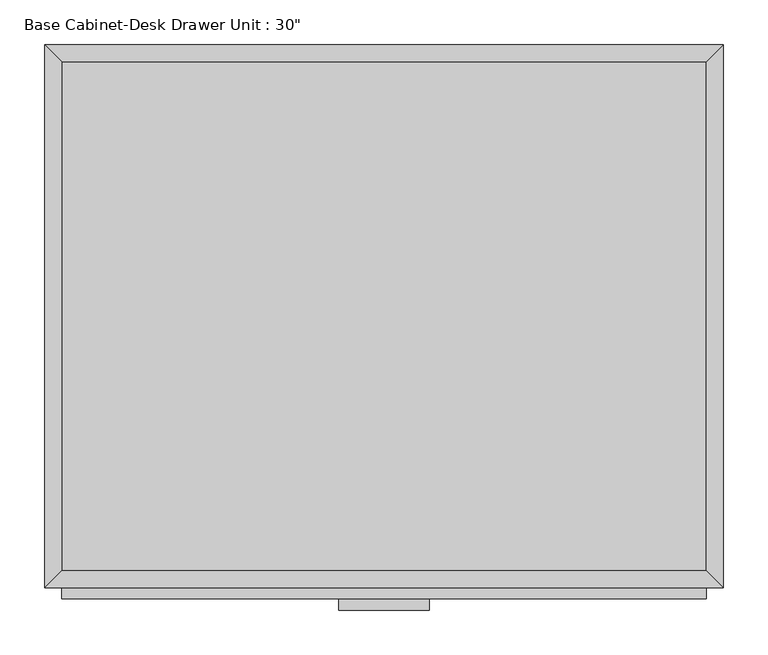
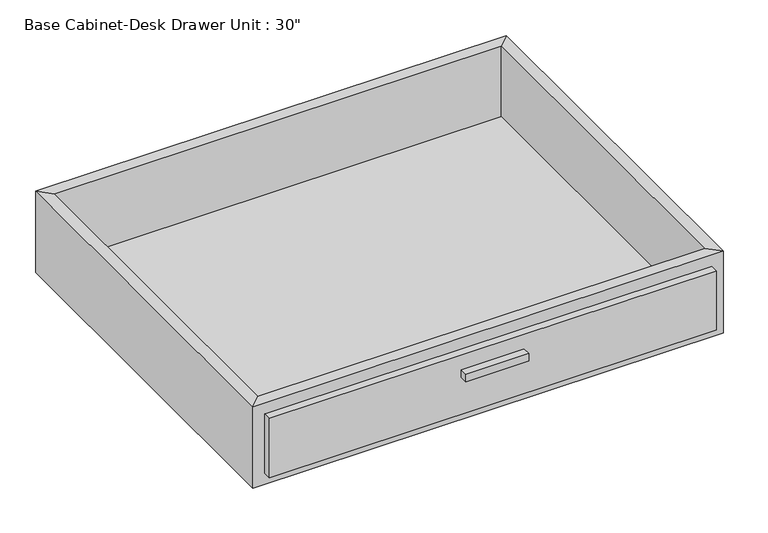
"""IFC4 building model written with IfcOpenShell, lengths in millimetres: furniture geometry."""

from ifc_helpers import new_model, si_unit, frame, origin, place, context, project, spatial, polyline, outline, extrude, faceted_brep, source, transform, mapped, element, save


def furniture_d895c99f(model_context):
    return source(origin(), model_context, "Body", "SolidModel", [
        extrude(outline(polyline([(69.5377049, -635.0), (-32.0622951, -635.0), (-32.0622951, -622.3), (69.5377049, -622.3), (69.5377049, -635.0)])), frame((0.0, 0.0, 819.15), z_axis=(0.0, 0.0, 1.0), x_axis=(1.0, 0.0, 0.0)), (0.0, 0.0, 1.0), 12.7),
        extrude(outline(polyline([(380.6877049, -622.3), (-343.2122951, -622.3), (-343.2122951, -609.6), (380.6877049, -609.6), (380.6877049, -622.3)])), frame((0.0, 0.0, 755.65), z_axis=(0.0, 0.0, 1.0), x_axis=(1.0, 0.0, 0.0)), (0.0, 0.0, 1.0), 101.6),
        extrude(outline(polyline([(380.6877049, -19.05), (380.6877049, -590.55), (-343.2122951, -590.55), (-343.2122951, -19.05), (380.6877049, -19.05)])), frame((0.0, 0.0, 736.6), z_axis=(0.0, 0.0, 1.0), x_axis=(1.0, 0.0, 0.0)), (0.0, 0.0, 1.0), 19.05),
        faceted_brep([(380.6877049, -590.55, 876.3), (380.6877049, -590.55, 736.6), (-343.2122951, -590.55, 736.6), (-343.2122951, -590.55, 876.3), (399.7377049, -609.6, 876.3), (-362.2622951, -609.6, 876.3), (399.7377049, -609.6, 736.6), (-362.2622951, -609.6, 736.6), (-343.2122951, -19.05, 736.6), (-343.2122951, -19.05, 876.3), (-362.2622951, 0.0, 876.3), (-362.2622951, 0.0, 736.6), (380.6877049, -19.05, 736.6), (380.6877049, -19.05, 876.3), (399.7377049, 0.0, 876.3), (399.7377049, 0.0, 736.6)], [[[0, 1, 2, 3]], [[4, 0, 3, 5]], [[6, 4, 5, 7]], [[1, 6, 7, 2]], [[3, 2, 8, 9]], [[5, 3, 9, 10]], [[7, 5, 10, 11]], [[2, 7, 11, 8]], [[9, 8, 12, 13]], [[10, 9, 13, 14]], [[11, 10, 14, 15]], [[8, 11, 15, 12]], [[13, 12, 1, 0]], [[14, 13, 0, 4]], [[15, 14, 4, 6]], [[12, 15, 6, 1]]]),
    ])


if __name__ == "__main__":
    model = new_model("IFC4")
    model_context = context("Model", 3, world=origin())
    ifc_project = project(units=[si_unit("LENGTHUNIT", "METRE", prefix="MILLI")], contexts=[model_context])
    site = spatial("IfcSite", under=ifc_project)
    building = spatial("IfcBuilding", under=site)
    placement = place(None, origin())
    furniture_shape = furniture_d895c99f(model_context)
    element("IfcFurniture", 1, ObjectType="Base Cabinet-Desk Drawer Unit : 30\"", at=placement, inside=building, context=model_context, shape_type="MappedRepresentation", body=[
        mapped(furniture_shape, transform((0.0, 0.0, 0.0), x_axis=(1.0, 0.0, 0.0), y_axis=(0.0, 1.0, 0.0), z_axis=(0.0, 0.0, 1.0))),
    ])
    save(model, "model.ifc")

# Revit data of these elements
# Type "Base Cabinet-Desk Drawer Unit : 30\""
#   Assembly Code = "C1030410"
#   Depth = 2' - 0"
#   Height = 2' - 10 1/2"
#   Width = 2' - 6"
#   Door/Drawer = Cabinets
#   Handles = Cabinets - Handles
#   Default Elevation = 0
# Element 1 (IfcFurniture, "Base Cabinet-Desk Drawer Unit : 30\"")
#   Materials on its faces: "Cabinets", "Cabinets - Handles"
# Materials
#   "Cabinets": class "Unassigned", colour RGB 249 249 249, transparency 0
#   "Cabinets - Handles": class "Unassigned", colour RGB 57 57 57, transparency 0
